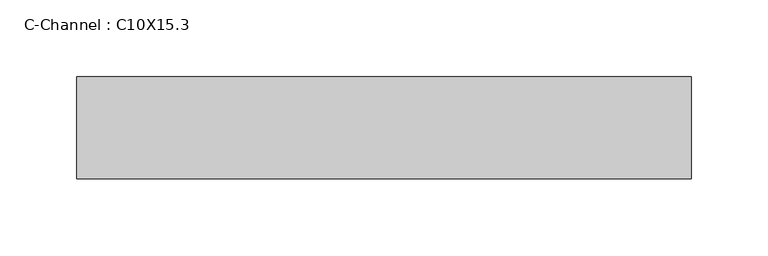
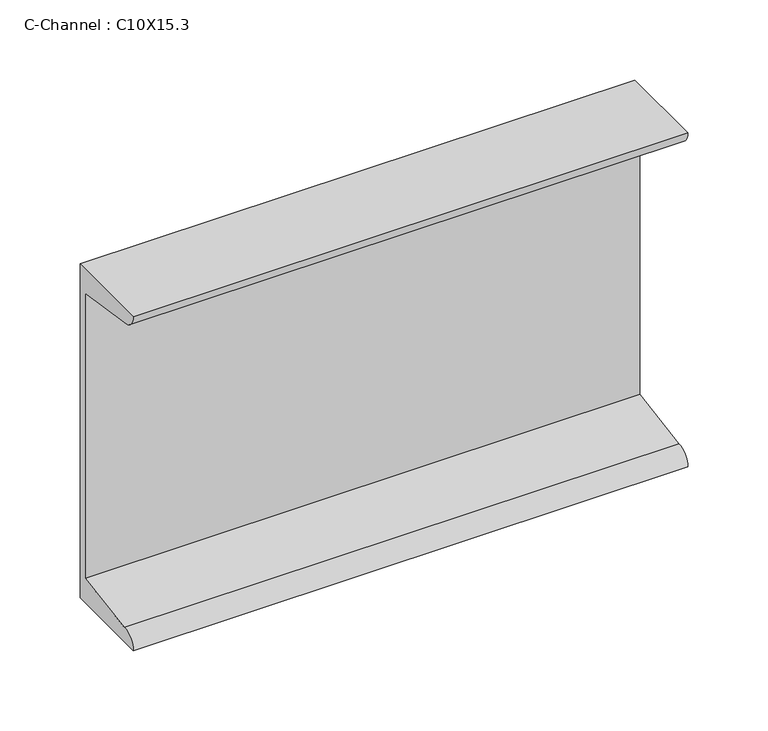
"""IFC4 building model written with IfcOpenShell, lengths in millimetres: beam geometry, C-Channel : C10X15.3."""

from ifc_helpers import new_model, si_unit, point, frame, frame_2d, origin, place, context, project, spatial, polyline, circle_curve, trimmed, segment, composite_curve, outline, extrude, source, transform, mapped, element, save


def c_channel_c10x15_3_6cbe0b48(model_context):
    return source(origin(), model_context, "Body", "SweptSolid", [
        extrude(outline(composite_curve([segment(polyline([(16.1036, 127.0), (16.1036, -127.0), (-49.9364, -127.0)]), True, "CONTINUOUS"), segment(trimmed(circle_curve(frame_2d((-38.862, -127.0)), 11.0744), [point((-49.9364, -127.0))], [point((-38.862, -115.9256))], False, "CARTESIAN"), True, "CONTINUOUS"), segment(polyline([(-38.862, -115.9256), (10.0076, -108.1854158), (10.0076, 108.1854158), (-38.862, 115.9256)]), True, "CONTINUOUS"), segment(trimmed(circle_curve(frame_2d((-38.862, 127.0)), 11.0744), [point((-38.862, 115.9256))], [point((-49.9364, 127.0))], False, "CARTESIAN"), True, "CONTINUOUS"), segment(polyline([(-49.9364, 127.0), (16.1036, 127.0)]), True, "CONTINUOUS")], self_intersect=False)), frame((-125.73, 0.0, 0.0), z_axis=(1.0, 0.0, 0.0), x_axis=(0.0, 1.0, 0.0)), (0.0, 0.0, 1.0), 398.78),
    ])


if __name__ == "__main__":
    model = new_model("IFC4")
    model_context = context("Model", 3, world=origin())
    ifc_project = project(units=[si_unit("LENGTHUNIT", "METRE", prefix="MILLI")], contexts=[model_context])
    site = spatial("IfcSite", under=ifc_project)
    building = spatial("IfcBuilding", under=site)
    placement = place(None, origin())
    c_channel_c10x15_3_shape = c_channel_c10x15_3_6cbe0b48(model_context)
    element("IfcBeam", 1, ObjectType="C-Channel : C10X15.3", at=placement, inside=building, context=model_context, shape_type="MappedRepresentation", body=[
        mapped(c_channel_c10x15_3_shape, transform((0.0, 0.0, 0.0), x_axis=(1.0, 0.0, 0.0), y_axis=(0.0, 1.0, 0.0), z_axis=(0.0, 0.0, 1.0))),
    ])
    save(model, "model.ifc")

# Revit data of these elements
# Type "C-Channel : C10X15.3"
#   Assembly Code = "B10"
#   W = 15.3
#   Length [instance default] = 5' - 0"
#   bf = 0' - 2.6"
#   d = 0' - 10"
#   tf = 0' - 0.436"
#   tw = 0' - 0.24"
#   x = 0' - 0.634"
#   A = 0.0311111 SF
#   Structural Material [instance default] = Steel ASTM A36
# Element 1 (IfcBeam, "C-Channel : C10X15.3")
#   Structural Material = Steel ASTM A992
#   Materials on its faces: "Steel ASTM A992"
# Materials
#   "Steel ASTM A36": class "Metal", colour RGB 199 199 199, transparency 0, Description = "Structural steel, ASTM A36 Grade B, mill finish", Cost = 0
#   "Steel ASTM A992": class "Metal", colour RGB 199 199 199, transparency 0, Description = "Structural steel 50ksi", Cost = 0
